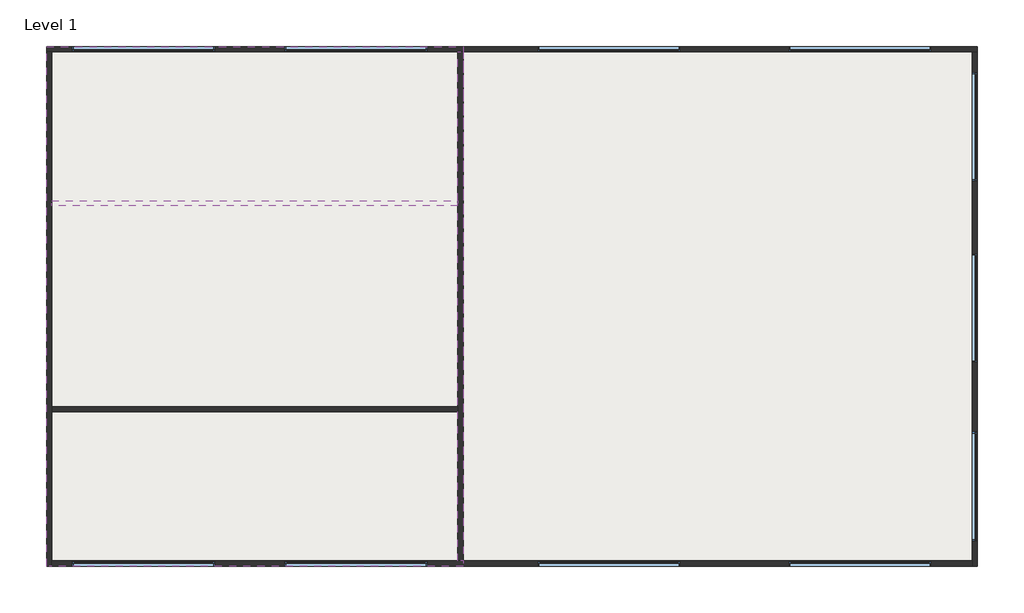
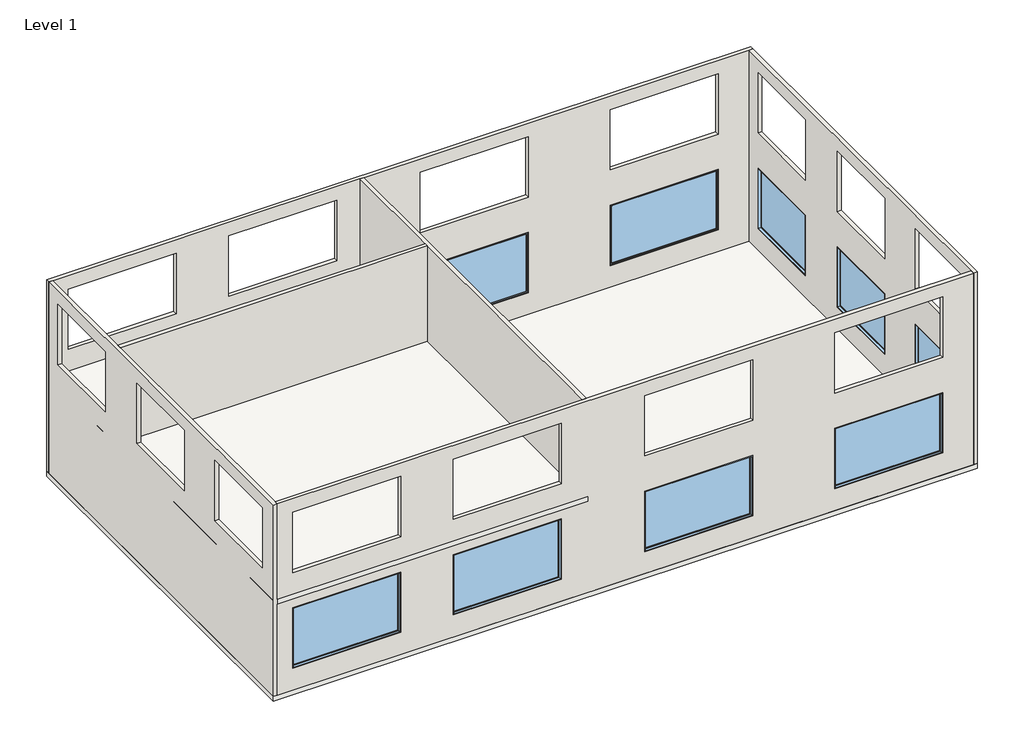
# One storey: 11 windows, 8 walls, 2 slabs.
"""IFC4 building model written with IfcOpenShell, lengths in millimetres."""

import ifcopenshell
import ifcopenshell.guid

model = None  # the IFC model being written
_history = None  # IfcOwnerHistory: only IFC2X3 demands one
_inside = {}  # id of a spatial element -> (the spatial element, [elements in it])
_under = {}  # id of a project, library or spatial element -> (it, [spatial elements below it])
_declared = {}  # id of a project -> (the project, [libraries it declares])
_typed = {}  # id of a type object -> (the type object, [elements of that type])
_made_of = {}  # id of a material, layer set ... -> (it, [elements and type objects made of it])


def new_model(schema):
    """Start an empty IFC model of exactly this schema.

    Asked for "IFC4X3", IfcOpenShell would pick the latest addendum, in which some entities
    have other attributes; the version numbers below select the first issue.
    IFC2X3 requires an IfcOwnerHistory on every rooted entity: one is made here for all.
    """
    global model, _history
    if schema == "IFC4X3":
        model = ifcopenshell.file(schema_version=(4, 3, 0, 0))
    else:
        model = ifcopenshell.file(schema=schema)
    _inside.clear()
    _under.clear()
    _declared.clear()
    _typed.clear()
    _made_of.clear()
    _history = None
    if model.schema == "IFC2X3":
        org = make("IfcOrganization", Name="unknown")
        user = make(
            "IfcPersonAndOrganization",
            ThePerson=make("IfcPerson", FamilyName="unknown"),
            TheOrganization=org,
        )
        app = make(
            "IfcApplication",
            ApplicationDeveloper=org,
            Version="unknown",
            ApplicationFullName="unknown",
            ApplicationIdentifier="unknown",
        )
        _history = make(
            "IfcOwnerHistory",
            OwningUser=user,
            OwningApplication=app,
            ChangeAction="ADDED",
            CreationDate=0,
        )
    return model


def make(cls, **values):
    """One entity of the class cls with the attributes given. An attribute that is None is left unset."""
    return model.create_entity(
        cls, **{name: value for name, value in values.items() if value is not None}
    )


def rooted(cls, **values):
    """An entity with a GlobalId (a new one), such as an element, a storey or a relation."""
    return make(cls, GlobalId=ifcopenshell.guid.new(), OwnerHistory=_history, **values)


def si_unit(unit_type, name, prefix=None):
    """IfcSIUnit, for example si_unit("LENGTHUNIT", "METRE", prefix="MILLI")."""
    return make("IfcSIUnit", UnitType=unit_type, Prefix=prefix, Name=name)


def assignment(units):
    """IfcUnitAssignment: the units of a project."""
    return None if units is None else make("IfcUnitAssignment", Units=units)


def point(xyz):
    """IfcCartesianPoint."""
    return None if xyz is None else make("IfcCartesianPoint", Coordinates=xyz)


def direction(xyz):
    """IfcDirection."""
    return None if xyz is None else make("IfcDirection", DirectionRatios=xyz)


def frame(location, z_axis=None, x_axis=None):
    """IfcAxis2Placement3D, a coordinate frame: its origin and axes. An axis left out is left unset."""
    return make(
        "IfcAxis2Placement3D",
        Location=point(location),
        Axis=direction(z_axis),
        RefDirection=direction(x_axis),
    )


def origin():
    """The frame at (0, 0, 0) with its axes left unset."""
    return frame((0.0, 0.0, 0.0))


def origin_with_axes():
    """The frame at (0, 0, 0) with the z axis (0, 0, 1) and the x axis (1, 0, 0) written out."""
    return frame((0.0, 0.0, 0.0), z_axis=(0.0, 0.0, 1.0), x_axis=(1.0, 0.0, 0.0))


def place(relative_to, where):
    """IfcLocalPlacement: puts the frame where relative to a parent placement (None: the world)."""
    return make(
        "IfcLocalPlacement", PlacementRelTo=relative_to, RelativePlacement=where
    )


def context(
    kind, dimensions, precision=None, world=None, true_north=None, identifier=None
):
    """IfcGeometricRepresentationContext, for example the 3D "Model" context."""
    return make(
        "IfcGeometricRepresentationContext",
        ContextIdentifier=identifier,
        ContextType=kind,
        CoordinateSpaceDimension=dimensions,
        Precision=precision,
        WorldCoordinateSystem=world,
        TrueNorth=true_north,
    )


def project(units=None, contexts=None):
    """IfcProject with its units and contexts."""
    return rooted(
        "IfcProject",
        Name="project",
        RepresentationContexts=contexts,
        UnitsInContext=assignment(units),
    )


def spatial(cls, under=None, at=None, **own):
    """A site, building, storey or space (cls), placed at a placement, below another one or the project."""
    s = rooted(cls, ObjectPlacement=at, **own)
    if under is not None:
        _under.setdefault(under.id(), (under, []))[1].append(s)
    return s


def polyline(points):
    """IfcPolyline through the points."""
    return make("IfcPolyline", Points=[point(p) for p in points])


def outline(outer, holes=None, kind="AREA"):
    """IfcArbitraryClosedProfileDef: a profile drawn as a closed curve; with holes, ...WithVoids."""
    if holes is None:
        return make("IfcArbitraryClosedProfileDef", ProfileType=kind, OuterCurve=outer)
    return make(
        "IfcArbitraryProfileDefWithVoids",
        ProfileType=kind,
        OuterCurve=outer,
        InnerCurves=holes,
    )


def extrude(swept, where, along, depth):
    """IfcExtrudedAreaSolid: the profile swept, set in the frame where, extruded along a direction by depth."""
    return make(
        "IfcExtrudedAreaSolid",
        SweptArea=swept,
        Position=where,
        ExtrudedDirection=direction(along),
        Depth=depth,
    )


def faces_of(points, faces, orient=None, outer=None):
    """IfcFace entities. A face is a list of loops; a loop is a list of indices into points, from 0.

    orient and outer hold one flag for each loop. By default every Orientation is true, the
    first loop of a face is its IfcFaceOuterBound and the others are IfcFaceBound.
    """
    made = []
    for i, loops in enumerate(faces):
        bounds = []
        for j, loop in enumerate(loops):
            is_outer = j == 0 if outer is None else outer[i][j]
            bounds.append(
                make(
                    "IfcFaceOuterBound" if is_outer else "IfcFaceBound",
                    Bound=make("IfcPolyLoop", Polygon=[points[k] for k in loop]),
                    Orientation=True if orient is None else orient[i][j],
                )
            )
        made.append(make("IfcFace", Bounds=bounds))
    return made


def faceted_brep(points, faces, orient=None, outer=None, voids=None):
    """IfcFacetedBrep: a solid bounded by flat faces; with voids (closed shells), ...WithVoids."""
    shared = [point(p) for p in points]
    hull = make("IfcClosedShell", CfsFaces=faces_of(shared, faces, orient, outer))
    if voids is None:
        return make("IfcFacetedBrep", Outer=hull)
    return make(
        "IfcFacetedBrepWithVoids",
        Outer=hull,
        Voids=[
            make(cls, CfsFaces=faces_of(shared, fs, o, b)) for cls, fs, o, b in voids
        ],
    )


def shape(context_of_items, identifier, shape_type, items):
    """IfcShapeRepresentation: the items that make up one representation, for example the "Body"."""
    return make(
        "IfcShapeRepresentation",
        ContextOfItems=context_of_items,
        RepresentationIdentifier=identifier,
        RepresentationType=shape_type,
        Items=items,
    )


def source(mapping_origin, context_of_items, identifier, shape_type, items):
    """IfcRepresentationMap: a shape defined once, which mapped items show again and again."""
    return make(
        "IfcRepresentationMap",
        MappingOrigin=mapping_origin,
        MappedRepresentation=shape(context_of_items, identifier, shape_type, items),
    )


def transform(
    local_origin,
    x_axis=None,
    y_axis=None,
    z_axis=None,
    scale=None,
    scale2=None,
    scale3=None,
    uniform=True,
):
    """IfcCartesianTransformationOperator3D, or its non-uniform kind. x_axis, y_axis, z_axis: its Axis1, 2, 3."""
    if uniform:
        return make(
            "IfcCartesianTransformationOperator3D",
            Axis1=direction(x_axis),
            Axis2=direction(y_axis),
            LocalOrigin=point(local_origin),
            Scale=scale,
            Axis3=direction(z_axis),
        )
    return make(
        "IfcCartesianTransformationOperator3DnonUniform",
        Axis1=direction(x_axis),
        Axis2=direction(y_axis),
        LocalOrigin=point(local_origin),
        Scale=scale,
        Axis3=direction(z_axis),
        Scale2=scale2,
        Scale3=scale3,
    )


def mapped(mapping_source, mapping_target):
    """IfcMappedItem: shows the shape of a source again, moved by a transform."""
    return make(
        "IfcMappedItem", MappingSource=mapping_source, MappingTarget=mapping_target
    )


def made_of(thing, what):
    """Note that an element or type object is made of a material, layer set ...; save() writes the relation."""
    if what is not None:
        _made_of.setdefault(what.id(), (what, []))[1].append(thing)
    return thing


def element(
    cls,
    number,
    at=None,
    inside=None,
    cuts=None,
    type_object=None,
    material=None,
    context=None,
    identifier="Body",
    shape_type=None,
    held_by="IfcProductDefinitionShape",
    body=None,
    shapes=None,
    **own,
):
    """One element of the class cls, such as IfcWall. Its Tag is "e" and its number.

    at: its placement. inside: the storey or other place that contains it. cuts: it is an
    opening in that element (IfcRelVoidsElement). A single representation is given by context,
    identifier, shape_type and body (its items); several are given by shapes. held_by: the class
    of the entity that holds the representations. save() writes the other relations.
    """
    e = rooted(cls, Tag="e%d" % number, ObjectPlacement=at, **own)
    if body is not None:
        shapes = [shape(context, identifier, shape_type, body)]
    if shapes is not None:
        e.Representation = make(held_by, Representations=shapes)
    if inside is not None:
        _inside.setdefault(inside.id(), (inside, []))[1].append(e)
    if cuts is not None:
        rooted(
            "IfcRelVoidsElement", RelatingBuildingElement=cuts, RelatedOpeningElement=e
        )
    if type_object is not None:
        _typed.setdefault(type_object.id(), (type_object, []))[1].append(e)
    return made_of(e, material)


def aggregate(whole, parts):
    """IfcRelAggregates: a whole, such as a stair, and the parts it consists of."""
    return rooted("IfcRelAggregates", RelatingObject=whole, RelatedObjects=parts)


def save(model, path):
    """Write the relations noted so far, then the file.

    IfcRelAggregates (storeys below a building ...), IfcRelContainedInSpatialStructure (elements
    in a storey), IfcRelDefinesByType, IfcRelAssociatesMaterial and IfcRelDeclares: one each for
    every whole, place, type object, material and project.
    """
    for whole, parts in _under.values():
        aggregate(whole, parts)
    for where, things in _inside.values():
        rooted(
            "IfcRelContainedInSpatialStructure",
            RelatedElements=things,
            RelatingStructure=where,
        )
    for kind, things in _typed.values():
        rooted("IfcRelDefinesByType", RelatedObjects=things, RelatingType=kind)
    for what, things in _made_of.values():
        rooted("IfcRelAssociatesMaterial", RelatedObjects=things, RelatingMaterial=what)
    for by, libraries in _declared.values():
        rooted("IfcRelDeclares", RelatingContext=by, RelatedDefinitions=libraries)
    model.write(path)


def m_fixed_2500x_4228mm_fd5e51e7(model_context):
    return source(origin(), model_context, "Body", "SweptSolid", [
        extrude(outline(polyline([(-2050.8, 54.2), (2050.8, 54.2), (2050.8, 42.2), (-2050.8, 42.2), (-2050.8, 54.2)])), frame((0.0, 0.0, 368.0), z_axis=(0.0, 0.0, 1.0), x_axis=(1.0, 0.0, 0.0)), (0.0, 0.0, 1.0), 2374.0),
        extrude(outline(polyline([(2786.0, -2094.8), (324.0, -2094.8), (324.0, 2094.8), (2786.0, 2094.8), (2786.0, -2094.8)]), holes=[polyline([(2742.0, -2050.8), (2742.0, 2050.8), (368.0, 2050.8), (368.0, -2050.8), (2742.0, -2050.8)])]), frame((0.0, 26.2, 0.0), z_axis=(0.0, 1.0, 0.0), x_axis=(0.0, 0.0, 1.0)), (0.0, 0.0, 1.0), 44.0),
        extrude(outline(polyline([(2805.0, -2113.8), (305.0, -2113.8), (305.0, 2113.8), (2805.0, 2113.8), (2805.0, -2113.8)]), holes=[polyline([(2786.0, -2094.8), (2786.0, 2094.8), (324.0, 2094.8), (324.0, -2094.8), (2786.0, -2094.8)])]), frame((0.0, 26.2, 0.0), z_axis=(0.0, 1.0, 0.0), x_axis=(0.0, 0.0, 1.0)), (0.0, 0.0, 1.0), 63.0),
        extrude(outline(polyline([(2805.0, -2113.8), (305.0, -2113.8), (305.0, 2113.8), (2805.0, 2113.8), (2805.0, -2113.8)]), holes=[polyline([(2773.0, -2081.8), (2773.0, 2081.8), (337.0, 2081.8), (337.0, -2081.8), (2773.0, -2081.8)])]), frame((0.0, -63.2, 0.0), z_axis=(0.0, 1.0, 0.0), x_axis=(0.0, 0.0, 1.0)), (0.0, 0.0, 1.0), 89.4),
    ])


def m_fixed_2500x_4228mm_f14c179f(model_context):
    return source(origin(), model_context, "Body", "SweptSolid", [
        extrude(outline(polyline([(-2050.8, -54.2), (-2050.8, -42.2), (2050.8, -42.2), (2050.8, -54.2), (-2050.8, -54.2)])), frame((0.0, 0.0, 368.0), z_axis=(0.0, 0.0, 1.0), x_axis=(1.0, 0.0, 0.0)), (0.0, 0.0, 1.0), 2374.0),
        extrude(outline(polyline([(2786.0, -2094.8), (324.0, -2094.8), (324.0, 2094.8), (2786.0, 2094.8), (2786.0, -2094.8)]), holes=[polyline([(2742.0, -2050.8), (2742.0, 2050.8), (368.0, 2050.8), (368.0, -2050.8), (2742.0, -2050.8)])]), frame((0.0, -70.2, 0.0), z_axis=(0.0, 1.0, 0.0), x_axis=(0.0, 0.0, 1.0)), (0.0, 0.0, 1.0), 44.0),
        extrude(outline(polyline([(2805.0, -2113.8), (305.0, -2113.8), (305.0, 2113.8), (2805.0, 2113.8), (2805.0, -2113.8)]), holes=[polyline([(2786.0, -2094.8), (2786.0, 2094.8), (324.0, 2094.8), (324.0, -2094.8), (2786.0, -2094.8)])]), frame((0.0, -89.2, 0.0), z_axis=(0.0, 1.0, 0.0), x_axis=(0.0, 0.0, 1.0)), (0.0, 0.0, 1.0), 63.0),
        extrude(outline(polyline([(2805.0, -2113.8), (305.0, -2113.8), (305.0, 2113.8), (2805.0, 2113.8), (2805.0, -2113.8)]), holes=[polyline([(2773.0, -2081.8), (2773.0, 2081.8), (337.0, 2081.8), (337.0, -2081.8), (2773.0, -2081.8)])]), frame((0.0, -26.2, 0.0), z_axis=(0.0, 1.0, 0.0), x_axis=(0.0, 0.0, 1.0)), (0.0, 0.0, 1.0), 89.4),
    ])


def m_fixed_2500x_3220mm_8b997f8c(model_context):
    return source(origin(), model_context, "Body", "SweptSolid", [
        extrude(outline(polyline([(-1546.8, -54.2), (-1546.8, -42.2), (1546.8, -42.2), (1546.8, -54.2), (-1546.8, -54.2)])), frame((0.0, 0.0, 368.0), z_axis=(0.0, 0.0, 1.0), x_axis=(1.0, 0.0, 0.0)), (0.0, 0.0, 1.0), 2374.0),
        extrude(outline(polyline([(2786.0, -1590.8), (324.0, -1590.8), (324.0, 1590.8), (2786.0, 1590.8), (2786.0, -1590.8)]), holes=[polyline([(2742.0, -1546.8), (2742.0, 1546.8), (368.0, 1546.8), (368.0, -1546.8), (2742.0, -1546.8)])]), frame((0.0, -70.2, 0.0), z_axis=(0.0, 1.0, 0.0), x_axis=(0.0, 0.0, 1.0)), (0.0, 0.0, 1.0), 44.0),
        extrude(outline(polyline([(2805.0, -1609.8), (305.0, -1609.8), (305.0, 1609.8), (2805.0, 1609.8), (2805.0, -1609.8)]), holes=[polyline([(2786.0, -1590.8), (2786.0, 1590.8), (324.0, 1590.8), (324.0, -1590.8), (2786.0, -1590.8)])]), frame((0.0, -89.2, 0.0), z_axis=(0.0, 1.0, 0.0), x_axis=(0.0, 0.0, 1.0)), (0.0, 0.0, 1.0), 63.0),
        extrude(outline(polyline([(2805.0, -1609.8), (305.0, -1609.8), (305.0, 1609.8), (2805.0, 1609.8), (2805.0, -1609.8)]), holes=[polyline([(2773.0, -1577.8), (2773.0, 1577.8), (337.0, 1577.8), (337.0, -1577.8), (2773.0, -1577.8)])]), frame((0.0, -26.2, 0.0), z_axis=(0.0, 1.0, 0.0), x_axis=(0.0, 0.0, 1.0)), (0.0, 0.0, 1.0), 89.4),
    ])


model = new_model("IFC4")

# Units and contexts
model_context = context("Model", 3, world=origin())
ifc_project = project(units=[si_unit("LENGTHUNIT", "METRE", prefix="MILLI")], contexts=[model_context])

# Site, building, storey
site = spatial("IfcSite", under=ifc_project)
building = spatial("IfcBuilding", under=site)
storey = spatial("IfcBuildingStorey", under=building, Name="Level 1", Elevation=0.0)

# Slabs
placement = place(None, origin())
element("IfcSlab", 1, ObjectType="160mm Concrete With 50mm Metal Deck", at=placement, inside=storey, context=model_context, shape_type="Brep", body=[
    faceted_brep([(29068.464681, 11296.9802217, -210.0), (29068.464681, -4095.4197783, -210.0), (1484.064681, -4095.4197783, -210.0), (1484.064681, 11296.9802217, -210.0), (29068.464681, 11296.9802217, 0.0), (1484.064681, 11296.9802217, 0.0), (1484.064681, -4095.4197783, 0.0), (28916.064681, -4095.4197783, 0.0), (29068.464681, -4095.4197783, 0.0), (29068.464681, 11144.5802217, 0.0)], [[[0, 1, 2, 3]], [[4, 5, 6, 7, 8, 9]], [[1, 0, 4, 9, 8]], [[2, 1, 8, 7, 6]], [[3, 2, 6, 5]], [[0, 3, 5, 4]]]),
])
element("IfcSlab", 2, ObjectType="160mm Concrete With 50mm Metal Deck", at=placement, inside=storey, context=model_context, shape_type="Brep", body=[
    faceted_brep([(13828.464681, 11296.9802217, 3752.4), (13828.464681, -3943.0197783, 3752.4), (13828.464681, -4095.4197783, 3752.4), (1636.464681, -4095.4197783, 3752.4), (1484.064681, -4095.4197783, 3752.4), (1484.064681, 11296.9802217, 3752.4), (13828.464681, 11296.9802217, 3962.4), (1484.064681, 11296.9802217, 3962.4), (1484.064681, -4095.4197783, 3962.4), (1636.464681, -4095.4197783, 3962.4), (13828.464681, -4095.4197783, 3962.4), (13828.464681, -3943.0197783, 3962.4)], [[[0, 1, 2, 3, 4, 5]], [[6, 7, 8, 9, 10, 11]], [[2, 1, 0, 6, 11, 10]], [[4, 3, 2, 10, 9, 8]], [[5, 4, 8, 7]], [[0, 5, 7, 6]]]),
])

# Walls
element("IfcWall", 3, ObjectType="Generic - 152.4mm", at=placement, inside=storey, context=model_context, shape_type="Brep", body=[
    faceted_brep([(1484.064681, 11144.5802217, 0.0), (1636.464681, 11144.5802217, 0.0), (13676.064681, 11144.5802217, 0.0), (13828.464681, 11144.5802217, 0.0), (28916.064681, 11144.5802217, 0.0), (29068.464681, 11144.5802217, 0.0), (29068.464681, 11144.5802217, 7924.8), (28916.064681, 11144.5802217, 7924.8), (13828.464681, 11144.5802217, 7924.8), (13676.064681, 11144.5802217, 7924.8), (1636.464681, 11144.5802217, 7924.8), (1484.064681, 11144.5802217, 7924.8), (6474.064681, 11144.5802217, 902.4), (2246.464681, 11144.5802217, 902.4), (2246.464681, 11144.5802217, 3402.4), (6474.064681, 11144.5802217, 3402.4), (12766.064681, 11144.5802217, 902.4), (8538.464681, 11144.5802217, 902.4), (8538.464681, 11144.5802217, 3402.4), (12766.064681, 11144.5802217, 3402.4), (20266.064681, 11144.5802217, 902.4), (16038.464681, 11144.5802217, 902.4), (16038.464681, 11144.5802217, 3402.4), (20266.064681, 11144.5802217, 3402.4), (27706.064681, 11144.5802217, 902.4), (23478.464681, 11144.5802217, 902.4), (23478.464681, 11144.5802217, 3402.4), (27706.064681, 11144.5802217, 3402.4), (27706.064681, 11144.5802217, 4862.4), (23478.464681, 11144.5802217, 4862.4), (23478.464681, 11144.5802217, 7362.4), (27706.064681, 11144.5802217, 7362.4), (20266.064681, 11144.5802217, 4862.4), (16038.464681, 11144.5802217, 4862.4), (16038.464681, 11144.5802217, 7362.4), (20266.064681, 11144.5802217, 7362.4), (12766.064681, 11144.5802217, 4862.4), (8538.464681, 11144.5802217, 4862.4), (8538.464681, 11144.5802217, 7362.4), (12766.064681, 11144.5802217, 7362.4), (6474.064681, 11144.5802217, 4862.4), (2246.464681, 11144.5802217, 4862.4), (2246.464681, 11144.5802217, 7362.4), (6474.064681, 11144.5802217, 7362.4), (1484.064681, 11296.9802217, 0.0), (1484.064681, 11296.9802217, 7924.8), (29068.464681, 11296.9802217, 7924.8), (29068.464681, 11296.9802217, 0.0), (6474.064681, 11296.9802217, 902.4), (6474.064681, 11296.9802217, 3402.4), (2246.464681, 11296.9802217, 3402.4), (2246.464681, 11296.9802217, 902.4), (12766.064681, 11296.9802217, 902.4), (12766.064681, 11296.9802217, 3402.4), (8538.464681, 11296.9802217, 3402.4), (8538.464681, 11296.9802217, 902.4), (20266.064681, 11296.9802217, 902.4), (20266.064681, 11296.9802217, 3402.4), (16038.464681, 11296.9802217, 3402.4), (16038.464681, 11296.9802217, 902.4), (27706.064681, 11296.9802217, 902.4), (27706.064681, 11296.9802217, 3402.4), (23478.464681, 11296.9802217, 3402.4), (23478.464681, 11296.9802217, 902.4), (27706.064681, 11296.9802217, 4862.4), (27706.064681, 11296.9802217, 7362.4), (23478.464681, 11296.9802217, 7362.4), (23478.464681, 11296.9802217, 4862.4), (20266.064681, 11296.9802217, 4862.4), (20266.064681, 11296.9802217, 7362.4), (16038.464681, 11296.9802217, 7362.4), (16038.464681, 11296.9802217, 4862.4), (12766.064681, 11296.9802217, 4862.4), (12766.064681, 11296.9802217, 7362.4), (8538.464681, 11296.9802217, 7362.4), (8538.464681, 11296.9802217, 4862.4), (6474.064681, 11296.9802217, 4862.4), (6474.064681, 11296.9802217, 7362.4), (2246.464681, 11296.9802217, 7362.4), (2246.464681, 11296.9802217, 4862.4)], [[[0, 1, 2, 3, 4, 5, 6, 7, 8, 9, 10, 11], [12, 13, 14, 15], [16, 17, 18, 19], [20, 21, 22, 23], [24, 25, 26, 27], [28, 29, 30, 31], [32, 33, 34, 35], [36, 37, 38, 39], [40, 41, 42, 43]], [[44, 45, 46, 47], [48, 49, 50, 51], [52, 53, 54, 55], [56, 57, 58, 59], [60, 61, 62, 63], [64, 65, 66, 67], [68, 69, 70, 71], [72, 73, 74, 75], [76, 77, 78, 79]], [[5, 4, 3, 2, 1, 0, 44, 47]], [[11, 10, 9, 8, 7, 6, 46, 45]], [[6, 5, 47, 46]], [[0, 11, 45, 44]], [[49, 48, 12, 15]], [[50, 49, 15, 14]], [[51, 50, 14, 13]], [[48, 51, 13, 12]], [[53, 52, 16, 19]], [[54, 53, 19, 18]], [[55, 54, 18, 17]], [[52, 55, 17, 16]], [[57, 56, 20, 23]], [[58, 57, 23, 22]], [[59, 58, 22, 21]], [[56, 59, 21, 20]], [[61, 60, 24, 27]], [[62, 61, 27, 26]], [[63, 62, 26, 25]], [[60, 63, 25, 24]], [[65, 64, 28, 31]], [[66, 65, 31, 30]], [[67, 66, 30, 29]], [[64, 67, 29, 28]], [[69, 68, 32, 35]], [[70, 69, 35, 34]], [[71, 70, 34, 33]], [[68, 71, 33, 32]], [[73, 72, 36, 39]], [[74, 73, 39, 38]], [[75, 74, 38, 37]], [[72, 75, 37, 36]], [[77, 76, 40, 43]], [[78, 77, 43, 42]], [[79, 78, 42, 41]], [[76, 79, 41, 40]]]),
])
element("IfcWall", 4, ObjectType="Generic - 152.4mm", at=placement, inside=storey, context=model_context, shape_type="Brep", body=[
    faceted_brep([(28916.064681, 11144.5802217, 0.0), (28916.064681, -3943.0197783, 0.0), (28916.064681, -4095.4197783, 0.0), (28916.064681, -4095.4197783, 7924.8), (28916.064681, -3943.0197783, 7924.8), (28916.064681, 11144.5802217, 7924.8), (28916.064681, -3343.0197783, 902.4), (28916.064681, -123.4197783, 902.4), (28916.064681, -123.4197783, 3402.4), (28916.064681, -3343.0197783, 3402.4), (28916.064681, 1942.9802217, 902.4), (28916.064681, 5162.5802217, 902.4), (28916.064681, 5162.5802217, 3402.4), (28916.064681, 1942.9802217, 3402.4), (28916.064681, 7310.9802217, 902.4), (28916.064681, 10530.5802217, 902.4), (28916.064681, 10530.5802217, 3402.4), (28916.064681, 7310.9802217, 3402.4), (28916.064681, -3343.0197783, 4864.8), (28916.064681, -123.4197783, 4864.8), (28916.064681, -123.4197783, 7364.8), (28916.064681, -3343.0197783, 7364.8), (28916.064681, 1942.9802217, 4864.8), (28916.064681, 5162.5802217, 4864.8), (28916.064681, 5162.5802217, 7364.8), (28916.064681, 1942.9802217, 7364.8), (28916.064681, 7310.9802217, 4864.8), (28916.064681, 10530.5802217, 4864.8), (28916.064681, 10530.5802217, 7364.8), (28916.064681, 7310.9802217, 7364.8), (29068.464681, 11144.5802217, 0.0), (29068.464681, 11144.5802217, 7924.8), (29068.464681, -4095.4197783, 7924.8), (29068.464681, -4095.4197783, 0.0), (29068.464681, -3343.0197783, 902.4), (29068.464681, -3343.0197783, 3402.4), (29068.464681, -123.4197783, 3402.4), (29068.464681, -123.4197783, 902.4), (29068.464681, 1942.9802217, 902.4), (29068.464681, 1942.9802217, 3402.4), (29068.464681, 5162.5802217, 3402.4), (29068.464681, 5162.5802217, 902.4), (29068.464681, 7310.9802217, 902.4), (29068.464681, 7310.9802217, 3402.4), (29068.464681, 10530.5802217, 3402.4), (29068.464681, 10530.5802217, 902.4), (29068.464681, -3343.0197783, 4864.8), (29068.464681, -3343.0197783, 7364.8), (29068.464681, -123.4197783, 7364.8), (29068.464681, -123.4197783, 4864.8), (29068.464681, 1942.9802217, 4864.8), (29068.464681, 1942.9802217, 7364.8), (29068.464681, 5162.5802217, 7364.8), (29068.464681, 5162.5802217, 4864.8), (29068.464681, 7310.9802217, 4864.8), (29068.464681, 7310.9802217, 7364.8), (29068.464681, 10530.5802217, 7364.8), (29068.464681, 10530.5802217, 4864.8)], [[[0, 1, 2, 3, 4, 5], [6, 7, 8, 9], [10, 11, 12, 13], [14, 15, 16, 17], [18, 19, 20, 21], [22, 23, 24, 25], [26, 27, 28, 29]], [[30, 31, 32, 33], [34, 35, 36, 37], [38, 39, 40, 41], [42, 43, 44, 45], [46, 47, 48, 49], [50, 51, 52, 53], [54, 55, 56, 57]], [[2, 1, 0, 30, 33]], [[5, 4, 3, 32, 31]], [[0, 5, 31, 30]], [[35, 34, 6, 9]], [[36, 35, 9, 8]], [[37, 36, 8, 7]], [[34, 37, 7, 6]], [[39, 38, 10, 13]], [[40, 39, 13, 12]], [[41, 40, 12, 11]], [[38, 41, 11, 10]], [[43, 42, 14, 17]], [[44, 43, 17, 16]], [[45, 44, 16, 15]], [[42, 45, 15, 14]], [[3, 2, 33, 32]], [[47, 46, 18, 21]], [[48, 47, 21, 20]], [[49, 48, 20, 19]], [[46, 49, 19, 18]], [[51, 50, 22, 25]], [[52, 51, 25, 24]], [[53, 52, 24, 23]], [[50, 53, 23, 22]], [[55, 54, 26, 29]], [[56, 55, 29, 28]], [[57, 56, 28, 27]], [[54, 57, 27, 26]]]),
])
element("IfcWall", 5, ObjectType="Generic - 152.4mm", at=placement, inside=storey, context=model_context, shape_type="Brep", body=[
    faceted_brep([(28916.064681, -3943.0197783, 0.0), (13828.464681, -3943.0197783, 0.0), (13676.064681, -3943.0197783, 0.0), (1636.464681, -3943.0197783, 0.0), (1636.464681, -3943.0197783, 3752.4), (13676.064681, -3943.0197783, 3752.4), (13828.464681, -3943.0197783, 3752.4), (13828.464681, -3943.0197783, 3962.4), (13676.064681, -3943.0197783, 3962.4), (1636.464681, -3943.0197783, 3962.4), (1636.464681, -3943.0197783, 7924.8), (13676.064681, -3943.0197783, 7924.8), (13828.464681, -3943.0197783, 7924.8), (28916.064681, -3943.0197783, 7924.8), (27706.064681, -3943.0197783, 902.4), (27706.064681, -3943.0197783, 3402.4), (23478.464681, -3943.0197783, 3402.4), (23478.464681, -3943.0197783, 902.4), (20266.064681, -3943.0197783, 902.4), (20266.064681, -3943.0197783, 3402.4), (16038.464681, -3943.0197783, 3402.4), (16038.464681, -3943.0197783, 902.4), (12766.064681, -3943.0197783, 902.4), (12766.064681, -3943.0197783, 3402.4), (8538.464681, -3943.0197783, 3402.4), (8538.464681, -3943.0197783, 902.4), (6474.064681, -3943.0197783, 902.4), (6474.064681, -3943.0197783, 3402.4), (2246.464681, -3943.0197783, 3402.4), (2246.464681, -3943.0197783, 902.4), (27706.064681, -3943.0197783, 4862.4), (27706.064681, -3943.0197783, 7362.4), (23478.464681, -3943.0197783, 7362.4), (23478.464681, -3943.0197783, 4862.4), (20266.064681, -3943.0197783, 4862.4), (20266.064681, -3943.0197783, 7362.4), (16038.464681, -3943.0197783, 7362.4), (16038.464681, -3943.0197783, 4862.4), (12766.064681, -3943.0197783, 4862.4), (12766.064681, -3943.0197783, 7362.4), (8538.464681, -3943.0197783, 7362.4), (8538.464681, -3943.0197783, 4862.4), (6474.064681, -3943.0197783, 4862.4), (6474.064681, -3943.0197783, 7362.4), (2246.464681, -3943.0197783, 7362.4), (2246.464681, -3943.0197783, 4862.4), (1636.464681, -4095.4197783, 0.0), (28916.064681, -4095.4197783, 0.0), (28916.064681, -4095.4197783, 7924.8), (1636.464681, -4095.4197783, 7924.8), (1636.464681, -4095.4197783, 3962.4), (13828.464681, -4095.4197783, 3962.4), (13828.464681, -4095.4197783, 3752.4), (1636.464681, -4095.4197783, 3752.4), (27706.064681, -4095.4197783, 3402.4), (27706.064681, -4095.4197783, 902.4), (23478.464681, -4095.4197783, 902.4), (23478.464681, -4095.4197783, 3402.4), (20266.064681, -4095.4197783, 3402.4), (20266.064681, -4095.4197783, 902.4), (16038.464681, -4095.4197783, 902.4), (16038.464681, -4095.4197783, 3402.4), (12766.064681, -4095.4197783, 3402.4), (12766.064681, -4095.4197783, 902.4), (8538.464681, -4095.4197783, 902.4), (8538.464681, -4095.4197783, 3402.4), (6474.064681, -4095.4197783, 3402.4), (6474.064681, -4095.4197783, 902.4), (2246.464681, -4095.4197783, 902.4), (2246.464681, -4095.4197783, 3402.4), (27706.064681, -4095.4197783, 7362.4), (27706.064681, -4095.4197783, 4862.4), (23478.464681, -4095.4197783, 4862.4), (23478.464681, -4095.4197783, 7362.4), (20266.064681, -4095.4197783, 7362.4), (20266.064681, -4095.4197783, 4862.4), (16038.464681, -4095.4197783, 4862.4), (16038.464681, -4095.4197783, 7362.4), (12766.064681, -4095.4197783, 7362.4), (12766.064681, -4095.4197783, 4862.4), (8538.464681, -4095.4197783, 4862.4), (8538.464681, -4095.4197783, 7362.4), (6474.064681, -4095.4197783, 7362.4), (6474.064681, -4095.4197783, 4862.4), (2246.464681, -4095.4197783, 4862.4), (2246.464681, -4095.4197783, 7362.4)], [[[0, 1, 2, 3, 4, 5, 6, 7, 8, 9, 10, 11, 12, 13], [14, 15, 16, 17], [18, 19, 20, 21], [22, 23, 24, 25], [26, 27, 28, 29], [30, 31, 32, 33], [34, 35, 36, 37], [38, 39, 40, 41], [42, 43, 44, 45]], [[46, 47, 48, 49, 50, 51, 52, 53], [54, 55, 56, 57], [58, 59, 60, 61], [62, 63, 64, 65], [66, 67, 68, 69], [70, 71, 72, 73], [74, 75, 76, 77], [78, 79, 80, 81], [82, 83, 84, 85]], [[3, 2, 1, 0, 47, 46]], [[13, 12, 11, 10, 49, 48]], [[15, 14, 55, 54]], [[16, 15, 54, 57]], [[17, 16, 57, 56]], [[14, 17, 56, 55]], [[19, 18, 59, 58]], [[20, 19, 58, 61]], [[21, 20, 61, 60]], [[18, 21, 60, 59]], [[23, 22, 63, 62]], [[24, 23, 62, 65]], [[25, 24, 65, 64]], [[22, 25, 64, 63]], [[27, 26, 67, 66]], [[28, 27, 66, 69]], [[29, 28, 69, 68]], [[26, 29, 68, 67]], [[47, 0, 13, 48]], [[3, 46, 53, 4]], [[49, 10, 9, 50]], [[31, 30, 71, 70]], [[32, 31, 70, 73]], [[33, 32, 73, 72]], [[30, 33, 72, 71]], [[35, 34, 75, 74]], [[36, 35, 74, 77]], [[37, 36, 77, 76]], [[34, 37, 76, 75]], [[39, 38, 79, 78]], [[40, 39, 78, 81]], [[41, 40, 81, 80]], [[38, 41, 80, 79]], [[43, 42, 83, 82]], [[44, 43, 82, 85]], [[45, 44, 85, 84]], [[42, 45, 84, 83]], [[52, 6, 5, 4, 53]], [[7, 51, 50, 9, 8]], [[6, 52, 51, 7]]]),
])
element("IfcWall", 6, ObjectType="Generic - 152.4mm", at=placement, inside=storey, context=model_context, shape_type="Brep", body=[
    faceted_brep([(1636.464681, -4095.4197783, 0.0), (1636.464681, -3943.0197783, 0.0), (1636.464681, 476.5802217, 0.0), (1636.464681, 628.9802217, 0.0), (1636.464681, 11144.5802217, 0.0), (1636.464681, 11144.5802217, 7924.8), (1636.464681, 6724.9802217, 7924.8), (1636.464681, 6572.5802217, 7924.8), (1636.464681, -3943.0197783, 7924.8), (1636.464681, -4095.4197783, 7924.8), (1636.464681, -4095.4197783, 3962.4), (1636.464681, -4095.4197783, 3752.4), (1636.464681, -3343.0197783, 4864.8), (1636.464681, -3343.0197783, 7364.8), (1636.464681, -123.4197783, 7364.8), (1636.464681, -123.4197783, 4864.8), (1636.464681, 1942.9802217, 4864.8), (1636.464681, 1942.9802217, 7364.8), (1636.464681, 5162.5802217, 7364.8), (1636.464681, 5162.5802217, 4864.8), (1636.464681, 7310.9802217, 4864.8), (1636.464681, 7310.9802217, 7364.8), (1636.464681, 10530.5802217, 7364.8), (1636.464681, 10530.5802217, 4864.8), (1484.064681, -4095.4197783, 0.0), (1484.064681, -4095.4197783, 7924.8), (1484.064681, 11144.5802217, 7924.8), (1484.064681, 11144.5802217, 0.0), (1484.064681, -3343.0197783, 4864.8), (1484.064681, -123.4197783, 4864.8), (1484.064681, -123.4197783, 7364.8), (1484.064681, -3343.0197783, 7364.8), (1484.064681, 1942.9802217, 4864.8), (1484.064681, 5162.5802217, 4864.8), (1484.064681, 5162.5802217, 7364.8), (1484.064681, 1942.9802217, 7364.8), (1484.064681, 7310.9802217, 4864.8), (1484.064681, 10530.5802217, 4864.8), (1484.064681, 10530.5802217, 7364.8), (1484.064681, 7310.9802217, 7364.8)], [[[0, 1, 2, 3, 4, 5, 6, 7, 8, 9, 10, 11], [12, 13, 14, 15], [16, 17, 18, 19], [20, 21, 22, 23]], [[24, 25, 26, 27], [28, 29, 30, 31], [32, 33, 34, 35], [36, 37, 38, 39]], [[4, 3, 2, 1, 0, 24, 27]], [[9, 8, 7, 6, 5, 26, 25]], [[5, 4, 27, 26]], [[0, 11, 10, 9, 25, 24]], [[13, 12, 28, 31]], [[14, 13, 31, 30]], [[15, 14, 30, 29]], [[12, 15, 29, 28]], [[17, 16, 32, 35]], [[18, 17, 35, 34]], [[19, 18, 34, 33]], [[16, 19, 33, 32]], [[21, 20, 36, 39]], [[22, 21, 39, 38]], [[23, 22, 38, 37]], [[20, 23, 37, 36]]]),
])
element("IfcWall", 7, ObjectType="Generic - 152.4mm - Interior", at=placement, inside=storey, context=model_context, shape_type="Brep", body=[
    faceted_brep([(13828.464681, -3943.0197783, 0.0), (13828.464681, 11144.5802217, 0.0), (13828.464681, 11144.5802217, 3752.4), (13828.464681, -3943.0197783, 3752.4), (13676.064681, -3943.0197783, 0.0), (13676.064681, -3943.0197783, 3752.4), (13676.064681, 476.5802217, 3752.4), (13676.064681, 628.9802217, 3752.4), (13676.064681, 11144.5802217, 3752.4), (13676.064681, 11144.5802217, 0.0), (13676.064681, 628.9802217, 0.0), (13676.064681, 476.5802217, 0.0)], [[[0, 1, 2, 3]], [[4, 5, 6, 7, 8, 9, 10, 11]], [[1, 0, 4, 11, 10, 9]], [[0, 3, 5, 4]], [[2, 1, 9, 8]], [[3, 2, 8, 7, 6, 5]]]),
])
element("IfcWall", 8, ObjectType="Generic - 152.4mm - Interior", at=placement, inside=storey, context=model_context, shape_type="SweptSolid", body=[
    extrude(outline(polyline([(1636.464681, 628.9802217), (13676.064681, 628.9802217), (13676.064681, 476.5802217), (1636.464681, 476.5802217), (1636.464681, 628.9802217)])), origin_with_axes(), (0.0, 0.0, 1.0), 3752.4),
])
element("IfcWall", 9, ObjectType="Generic - 152.4mm - Interior", at=placement, inside=storey, context=model_context, shape_type="Brep", body=[
    faceted_brep([(13676.064681, 11144.5802217, 3962.4), (13676.064681, 6724.9802217, 3962.4), (13676.064681, 6572.5802217, 3962.4), (13676.064681, -3943.0197783, 3962.4), (13676.064681, -3943.0197783, 7924.8), (13676.064681, 6572.5802217, 7924.8), (13676.064681, 6724.9802217, 7924.8), (13676.064681, 11144.5802217, 7924.8), (13828.464681, 11144.5802217, 3962.4), (13828.464681, 11144.5802217, 7924.8), (13828.464681, -3943.0197783, 7924.8), (13828.464681, -3943.0197783, 3962.4)], [[[0, 1, 2, 3, 4, 5, 6, 7]], [[8, 9, 10, 11]], [[3, 2, 1, 0, 8, 11]], [[7, 6, 5, 4, 10, 9]], [[4, 3, 11, 10]], [[0, 7, 9, 8]]]),
])
element("IfcWall", 10, ObjectType="Generic - 152.4mm - Interior", at=placement, inside=storey, context=model_context, shape_type="SweptSolid", body=[
    extrude(outline(polyline([(1636.464681, 6724.9802217), (13676.064681, 6724.9802217), (13676.064681, 6572.5802217), (1636.464681, 6572.5802217), (1636.464681, 6724.9802217)])), frame((0.0, 0.0, 3962.4), z_axis=(0.0, 0.0, 1.0), x_axis=(1.0, 0.0, 0.0)), (0.0, 0.0, 1.0), 3962.4),
])

# Windows
m_fixed_2500x_4228mm_shape = m_fixed_2500x_4228mm_fd5e51e7(model_context)
element("IfcWindow", 11, ObjectType="M_Fixed : 2500X 4228mm", at=placement, inside=storey, context=model_context, shape_type="MappedRepresentation", body=[
    mapped(m_fixed_2500x_4228mm_shape, transform((4360.264681, 11233.7802217, 597.4), x_axis=(-1.0, 0.0, 0.0), y_axis=(0.0, -1.0, 0.0), z_axis=(0.0, 0.0, 1.0))),
])
element("IfcWindow", 12, ObjectType="M_Fixed : 2500X 4228mm", at=placement, inside=storey, context=model_context, shape_type="MappedRepresentation", body=[
    mapped(m_fixed_2500x_4228mm_shape, transform((10652.264681, 11233.7802217, 597.4), x_axis=(-1.0, 0.0, 0.0), y_axis=(0.0, -1.0, 0.0), z_axis=(0.0, 0.0, 1.0))),
])
element("IfcWindow", 13, ObjectType="M_Fixed : 2500X 4228mm", at=placement, inside=storey, context=model_context, shape_type="MappedRepresentation", body=[
    mapped(m_fixed_2500x_4228mm_shape, transform((18152.264681, 11233.7802217, 597.4), x_axis=(-1.0, 0.0, 0.0), y_axis=(0.0, -1.0, 0.0), z_axis=(0.0, 0.0, 1.0))),
])
element("IfcWindow", 14, ObjectType="M_Fixed : 2500X 4228mm", at=placement, inside=storey, context=model_context, shape_type="MappedRepresentation", body=[
    mapped(m_fixed_2500x_4228mm_shape, transform((25592.264681, 11233.7802217, 597.4), x_axis=(-1.0, 0.0, 0.0), y_axis=(0.0, -1.0, 0.0), z_axis=(0.0, 0.0, 1.0))),
])
m_fixed_2500x_4228mm_2_shape = m_fixed_2500x_4228mm_f14c179f(model_context)
element("IfcWindow", 15, ObjectType="M_Fixed : 2500X 4228mm", at=placement, inside=storey, context=model_context, shape_type="MappedRepresentation", body=[
    mapped(m_fixed_2500x_4228mm_2_shape, transform((4360.264681, -4032.2197783, 597.4), x_axis=(-1.0, 0.0, 0.0), y_axis=(0.0, -1.0, 0.0), z_axis=(0.0, 0.0, 1.0))),
])
element("IfcWindow", 16, ObjectType="M_Fixed : 2500X 4228mm", at=placement, inside=storey, context=model_context, shape_type="MappedRepresentation", body=[
    mapped(m_fixed_2500x_4228mm_2_shape, transform((10652.264681, -4032.2197783, 597.4), x_axis=(-1.0, 0.0, 0.0), y_axis=(0.0, -1.0, 0.0), z_axis=(0.0, 0.0, 1.0))),
])
element("IfcWindow", 17, ObjectType="M_Fixed : 2500X 4228mm", at=placement, inside=storey, context=model_context, shape_type="MappedRepresentation", body=[
    mapped(m_fixed_2500x_4228mm_2_shape, transform((18152.264681, -4032.2197783, 597.4), x_axis=(-1.0, 0.0, 0.0), y_axis=(0.0, -1.0, 0.0), z_axis=(0.0, 0.0, 1.0))),
])
element("IfcWindow", 18, ObjectType="M_Fixed : 2500X 4228mm", at=placement, inside=storey, context=model_context, shape_type="MappedRepresentation", body=[
    mapped(m_fixed_2500x_4228mm_2_shape, transform((25592.264681, -4032.2197783, 597.4), x_axis=(-1.0, 0.0, 0.0), y_axis=(0.0, -1.0, 0.0), z_axis=(0.0, 0.0, 1.0))),
])
m_fixed_2500x_3220mm_shape = m_fixed_2500x_3220mm_8b997f8c(model_context)
element("IfcWindow", 19, ObjectType="M_Fixed : 2500x 3220mm", at=placement, inside=storey, context=model_context, shape_type="MappedRepresentation", body=[
    mapped(m_fixed_2500x_3220mm_shape, transform((28979.264681, 8920.7802217, 597.4), x_axis=(0.0, 1.0, 0.0), y_axis=(-1.0, 0.0, 0.0), z_axis=(0.0, 0.0, 1.0))),
])
element("IfcWindow", 20, ObjectType="M_Fixed : 2500x 3220mm", at=placement, inside=storey, context=model_context, shape_type="MappedRepresentation", body=[
    mapped(m_fixed_2500x_3220mm_shape, transform((28979.264681, 3552.7802217, 597.4), x_axis=(0.0, 1.0, 0.0), y_axis=(-1.0, 0.0, 0.0), z_axis=(0.0, 0.0, 1.0))),
])
element("IfcWindow", 21, ObjectType="M_Fixed : 2500x 3220mm", at=placement, inside=storey, context=model_context, shape_type="MappedRepresentation", body=[
    mapped(m_fixed_2500x_3220mm_shape, transform((28979.264681, -1733.2197783, 597.4), x_axis=(0.0, 1.0, 0.0), y_axis=(-1.0, 0.0, 0.0), z_axis=(0.0, 0.0, 1.0))),
])

save(model, "model.ifc")

# Revit data of these elements
# Project information
#   Project Issue Date = "Issue Date"
#   Project Status = "Project Status"
#   Client Name = "Owner"
#   Project Address = "Enter address here"
#   Project Name = "Project Name"
#   Project Number = "Project Number"
# Type "160mm Concrete With 50mm Metal Deck"
#   Function = 0
#   Layers, outside or top first: 210 mm no material (function 1); 0 mm "Metal Deck" (function 200)
# Type "Generic - 152.4mm"
#   Layers, outside or top first: 152.4 mm no material (function 1)
# Type "Generic - 152.4mm - Interior"
#   Layers, outside or top first: 152.4 mm no material (function 1)
# Type "M_Fixed : 2500X 4228mm"
#   Type Mark = "25"
#   Height = 2500 mm
#   Default Sill Height = 305 mm
#   Width = 4227.6 mm
#   Window Inset = 19 mm
#   Frame Exterior Material = Sash
#   Frame Interior Material = Sash
#   Glass Pane Material = Glass
#   Sash = Sash
#   Wall Closure = (empty or 0)
# Type "M_Fixed : 2500x 3220mm"
#   Type Mark = "26"
#   Height = 2500 mm
#   Default Sill Height = 305 mm
#   Width = 3219.6 mm
#   Window Inset = 19 mm
#   Frame Exterior Material = Sash
#   Frame Interior Material = Sash
#   Glass Pane Material = Glass
#   Sash = Sash
#   Wall Closure = (empty or 0)
# Element 1 (IfcSlab, "160mm Concrete With 50mm Metal Deck")
#   Height Offset From Level = 0 mm
#   Phase Created = New Construction
#   Materials on its faces: "Metal Deck", "Default Floor"
# Element 2 (IfcSlab, "160mm Concrete With 50mm Metal Deck")
#   Height Offset From Level = 3962.4 mm
#   Phase Created = New Construction
#   Materials on its faces: "Metal Deck", "Default Floor"
# Elements 3, 4, 5, 6 (IfcWall, "Generic - 152.4mm")
#   Top Offset = 0 mm
#   Base Offset = 0 mm
#   wall height = 7924.8 mm
#   Phase Created = New Construction
#   Base Constraint = Level 1
#   Top Constraint = Roof Level
#   Materials on its faces: "Default Wall"
# Element 7 (IfcWall, "Generic - 152.4mm - Interior")
#   Top Offset = 3962.4 mm
#   Base Offset = 0 mm
#   wall height = 3752.4 mm
#   Phase Created = New Construction
#   Base Constraint = Level 1
#   Top Constraint = Level 1
#   Materials on its faces: "Default Wall"
# Element 8 (IfcWall, "Generic - 152.4mm - Interior")
#   Top Offset = 3862.4 mm
#   Base Offset = 0 mm
#   wall height = 3752.4 mm
#   Phase Created = New Construction
#   Base Constraint = Level 1
#   Top Constraint = Level 1
#   Materials on its faces: "Default Wall"
# Elements 9, 10 (IfcWall, "Generic - 152.4mm - Interior")
#   built-in parameter 1001111 = 3962.4 mm
#   Top Offset = 0 mm
#   Base Offset = 3962.4 mm
#   Unconnected Height = 3962.4 mm
#   wall height = 3962.4 mm
#   Phase Created = New Construction
#   Base Constraint = Level 1
#   Top Constraint = Roof Level
#   Materials on its faces: "Default Wall"
# Element 11 (IfcWindow, "M_Fixed : 2500X 4228mm")
#   Mark = "10"
#   Phase Created = New Construction
#   Materials on its faces: "Sash", "Glass"
# Element 12 (IfcWindow, "M_Fixed : 2500X 4228mm")
#   Mark = "11"
#   Phase Created = New Construction
#   Materials on its faces: "Sash", "Glass"
# Element 13 (IfcWindow, "M_Fixed : 2500X 4228mm")
#   Mark = "12"
#   Phase Created = New Construction
#   Materials on its faces: "Sash", "Glass"
# Element 14 (IfcWindow, "M_Fixed : 2500X 4228mm")
#   Mark = "13"
#   Phase Created = New Construction
#   Materials on its faces: "Sash", "Glass"
# Element 15 (IfcWindow, "M_Fixed : 2500X 4228mm")
#   Mark = "14"
#   Phase Created = New Construction
#   Materials on its faces: "Sash", "Glass"
# Element 16 (IfcWindow, "M_Fixed : 2500X 4228mm")
#   Mark = "15"
#   Phase Created = New Construction
#   Materials on its faces: "Sash", "Glass"
# Element 17 (IfcWindow, "M_Fixed : 2500X 4228mm")
#   Mark = "16"
#   Phase Created = New Construction
#   Materials on its faces: "Sash", "Glass"
# Element 18 (IfcWindow, "M_Fixed : 2500X 4228mm")
#   Mark = "17"
#   Phase Created = New Construction
#   Materials on its faces: "Sash", "Glass"
# Element 19 (IfcWindow, "M_Fixed : 2500x 3220mm")
#   Mark = "30"
#   Phase Created = New Construction
#   Materials on its faces: "Sash", "Glass"
# Element 20 (IfcWindow, "M_Fixed : 2500x 3220mm")
#   Mark = "31"
#   Phase Created = New Construction
#   Materials on its faces: "Sash", "Glass"
# Element 21 (IfcWindow, "M_Fixed : 2500x 3220mm")
#   Mark = "32"
#   Phase Created = New Construction
#   Materials on its faces: "Sash", "Glass"
# Materials
#   "Metal Deck": class "Metal", colour RGB 247 247 247, transparency 0, Description = "Steel, mill finish", Cost = 0
#   "Sash": class "Wood", colour RGB 136 99 55, transparency 0
#   "Glass": class "Glass", colour RGB 0 128 192, transparency 0.9, Description = "Soda Lime Glass", Cost = 0
#   "Default Floor": class "Miscellaneous", colour RGB 127 127 127, transparency 0, Cost = 0
#   "Default Wall": class "Miscellaneous", colour RGB 128 128 128, transparency 0, Cost = 0
# Room at (7259.725, -1600.456) mm, phase "New Construction", upper level "Level 2", upper offset 0 mm, lower offset 0 mm
#   Number = "6"
#   Name = "Room"
# Room at (8198.725, 4816.984) mm, phase "New Construction", upper level "Level 2", upper offset 0 mm, lower offset 0 mm
#   Number = "7"
#   Name = "Room"
# Room at (21274.823, 2677.837) mm, phase "New Construction", upper level "Roof Level", upper offset 0 mm, lower offset 0 mm
#   Number = "8"
#   Name = "Room"
